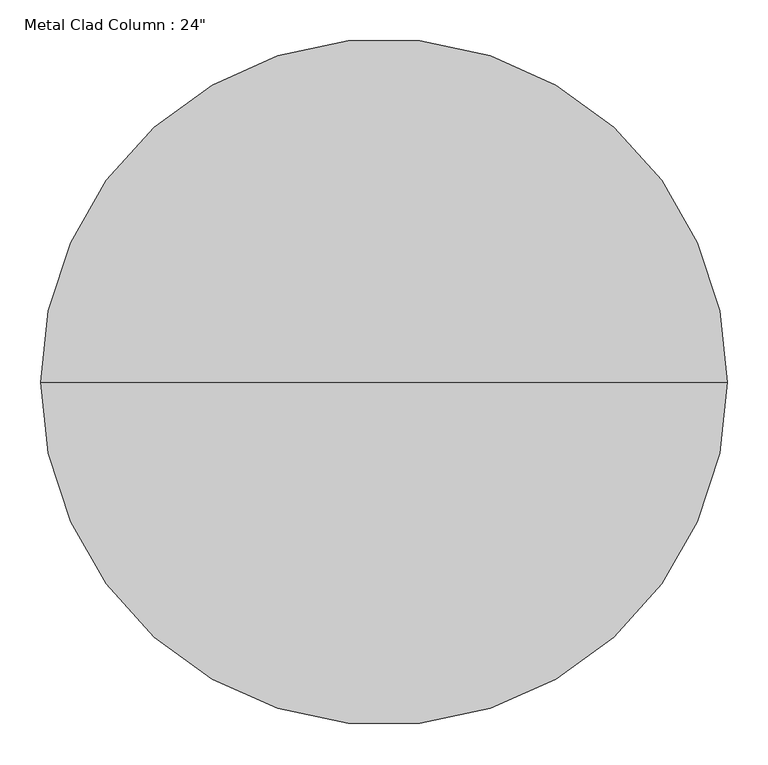
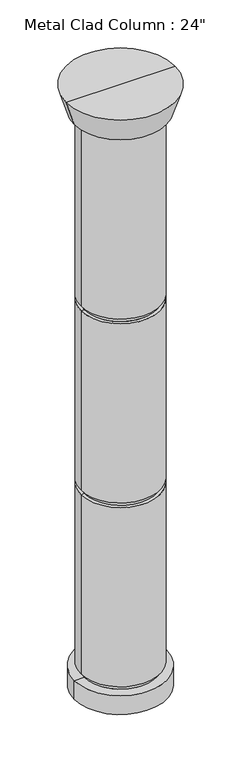
"""IFC4 building model written with IfcOpenShell, lengths in millimetres: column geometry."""

import ifcopenshell
import ifcopenshell.guid

model = None  # the IFC model being written
_history = None  # IfcOwnerHistory: only IFC2X3 demands one
_inside = {}  # id of a spatial element -> (the spatial element, [elements in it])
_under = {}  # id of a project, library or spatial element -> (it, [spatial elements below it])
_declared = {}  # id of a project -> (the project, [libraries it declares])
_typed = {}  # id of a type object -> (the type object, [elements of that type])
_made_of = {}  # id of a material, layer set ... -> (it, [elements and type objects made of it])


def new_model(schema):
    """Start an empty IFC model of exactly this schema.

    Asked for "IFC4X3", IfcOpenShell would pick the latest addendum, in which some entities
    have other attributes; the version numbers below select the first issue.
    IFC2X3 requires an IfcOwnerHistory on every rooted entity: one is made here for all.
    """
    global model, _history
    if schema == "IFC4X3":
        model = ifcopenshell.file(schema_version=(4, 3, 0, 0))
    else:
        model = ifcopenshell.file(schema=schema)
    _inside.clear()
    _under.clear()
    _declared.clear()
    _typed.clear()
    _made_of.clear()
    _history = None
    if model.schema == "IFC2X3":
        org = make("IfcOrganization", Name="unknown")
        user = make(
            "IfcPersonAndOrganization",
            ThePerson=make("IfcPerson", FamilyName="unknown"),
            TheOrganization=org,
        )
        app = make(
            "IfcApplication",
            ApplicationDeveloper=org,
            Version="unknown",
            ApplicationFullName="unknown",
            ApplicationIdentifier="unknown",
        )
        _history = make(
            "IfcOwnerHistory",
            OwningUser=user,
            OwningApplication=app,
            ChangeAction="ADDED",
            CreationDate=0,
        )
    return model


def make(cls, **values):
    """One entity of the class cls with the attributes given. An attribute that is None is left unset."""
    return model.create_entity(
        cls, **{name: value for name, value in values.items() if value is not None}
    )


def rooted(cls, **values):
    """An entity with a GlobalId (a new one), such as an element, a storey or a relation."""
    return make(cls, GlobalId=ifcopenshell.guid.new(), OwnerHistory=_history, **values)


def si_unit(unit_type, name, prefix=None):
    """IfcSIUnit, for example si_unit("LENGTHUNIT", "METRE", prefix="MILLI")."""
    return make("IfcSIUnit", UnitType=unit_type, Prefix=prefix, Name=name)


def assignment(units):
    """IfcUnitAssignment: the units of a project."""
    return None if units is None else make("IfcUnitAssignment", Units=units)


def point(xyz):
    """IfcCartesianPoint."""
    return None if xyz is None else make("IfcCartesianPoint", Coordinates=xyz)


def direction(xyz):
    """IfcDirection."""
    return None if xyz is None else make("IfcDirection", DirectionRatios=xyz)


def frame(location, z_axis=None, x_axis=None):
    """IfcAxis2Placement3D, a coordinate frame: its origin and axes. An axis left out is left unset."""
    return make(
        "IfcAxis2Placement3D",
        Location=point(location),
        Axis=direction(z_axis),
        RefDirection=direction(x_axis),
    )


def origin():
    """The frame at (0, 0, 0) with its axes left unset."""
    return frame((0.0, 0.0, 0.0))


def place(relative_to, where):
    """IfcLocalPlacement: puts the frame where relative to a parent placement (None: the world)."""
    return make(
        "IfcLocalPlacement", PlacementRelTo=relative_to, RelativePlacement=where
    )


def context(
    kind, dimensions, precision=None, world=None, true_north=None, identifier=None
):
    """IfcGeometricRepresentationContext, for example the 3D "Model" context."""
    return make(
        "IfcGeometricRepresentationContext",
        ContextIdentifier=identifier,
        ContextType=kind,
        CoordinateSpaceDimension=dimensions,
        Precision=precision,
        WorldCoordinateSystem=world,
        TrueNorth=true_north,
    )


def project(units=None, contexts=None):
    """IfcProject with its units and contexts."""
    return rooted(
        "IfcProject",
        Name="project",
        RepresentationContexts=contexts,
        UnitsInContext=assignment(units),
    )


def spatial(cls, under=None, at=None, **own):
    """A site, building, storey or space (cls), placed at a placement, below another one or the project."""
    s = rooted(cls, ObjectPlacement=at, **own)
    if under is not None:
        _under.setdefault(under.id(), (under, []))[1].append(s)
    return s


def polyline(points):
    """IfcPolyline through the points."""
    return make("IfcPolyline", Points=[point(p) for p in points])


def circle_curve(where, radius):
    """IfcCircle in the frame where."""
    return make("IfcCircle", Position=where, Radius=radius)


def shape(context_of_items, identifier, shape_type, items):
    """IfcShapeRepresentation: the items that make up one representation, for example the "Body"."""
    return make(
        "IfcShapeRepresentation",
        ContextOfItems=context_of_items,
        RepresentationIdentifier=identifier,
        RepresentationType=shape_type,
        Items=items,
    )


def source(mapping_origin, context_of_items, identifier, shape_type, items):
    """IfcRepresentationMap: a shape defined once, which mapped items show again and again."""
    return make(
        "IfcRepresentationMap",
        MappingOrigin=mapping_origin,
        MappedRepresentation=shape(context_of_items, identifier, shape_type, items),
    )


def transform(
    local_origin,
    x_axis=None,
    y_axis=None,
    z_axis=None,
    scale=None,
    scale2=None,
    scale3=None,
    uniform=True,
):
    """IfcCartesianTransformationOperator3D, or its non-uniform kind. x_axis, y_axis, z_axis: its Axis1, 2, 3."""
    if uniform:
        return make(
            "IfcCartesianTransformationOperator3D",
            Axis1=direction(x_axis),
            Axis2=direction(y_axis),
            LocalOrigin=point(local_origin),
            Scale=scale,
            Axis3=direction(z_axis),
        )
    return make(
        "IfcCartesianTransformationOperator3DnonUniform",
        Axis1=direction(x_axis),
        Axis2=direction(y_axis),
        LocalOrigin=point(local_origin),
        Scale=scale,
        Axis3=direction(z_axis),
        Scale2=scale2,
        Scale3=scale3,
    )


def mapped(mapping_source, mapping_target):
    """IfcMappedItem: shows the shape of a source again, moved by a transform."""
    return make(
        "IfcMappedItem", MappingSource=mapping_source, MappingTarget=mapping_target
    )


def made_of(thing, what):
    """Note that an element or type object is made of a material, layer set ...; save() writes the relation."""
    if what is not None:
        _made_of.setdefault(what.id(), (what, []))[1].append(thing)
    return thing


def element(
    cls,
    number,
    at=None,
    inside=None,
    cuts=None,
    type_object=None,
    material=None,
    context=None,
    identifier="Body",
    shape_type=None,
    held_by="IfcProductDefinitionShape",
    body=None,
    shapes=None,
    **own,
):
    """One element of the class cls, such as IfcWall. Its Tag is "e" and its number.

    at: its placement. inside: the storey or other place that contains it. cuts: it is an
    opening in that element (IfcRelVoidsElement). A single representation is given by context,
    identifier, shape_type and body (its items); several are given by shapes. held_by: the class
    of the entity that holds the representations. save() writes the other relations.
    """
    e = rooted(cls, Tag="e%d" % number, ObjectPlacement=at, **own)
    if body is not None:
        shapes = [shape(context, identifier, shape_type, body)]
    if shapes is not None:
        e.Representation = make(held_by, Representations=shapes)
    if inside is not None:
        _inside.setdefault(inside.id(), (inside, []))[1].append(e)
    if cuts is not None:
        rooted(
            "IfcRelVoidsElement", RelatingBuildingElement=cuts, RelatedOpeningElement=e
        )
    if type_object is not None:
        _typed.setdefault(type_object.id(), (type_object, []))[1].append(e)
    return made_of(e, material)


def aggregate(whole, parts):
    """IfcRelAggregates: a whole, such as a stair, and the parts it consists of."""
    return rooted("IfcRelAggregates", RelatingObject=whole, RelatedObjects=parts)


def save(model, path):
    """Write the relations noted so far, then the file.

    IfcRelAggregates (storeys below a building ...), IfcRelContainedInSpatialStructure (elements
    in a storey), IfcRelDefinesByType, IfcRelAssociatesMaterial and IfcRelDeclares: one each for
    every whole, place, type object, material and project.
    """
    for whole, parts in _under.values():
        aggregate(whole, parts)
    for where, things in _inside.values():
        rooted(
            "IfcRelContainedInSpatialStructure",
            RelatedElements=things,
            RelatingStructure=where,
        )
    for kind, things in _typed.values():
        rooted("IfcRelDefinesByType", RelatedObjects=things, RelatingType=kind)
    for what, things in _made_of.values():
        rooted("IfcRelAssociatesMaterial", RelatedObjects=things, RelatingMaterial=what)
    for by, libraries in _declared.values():
        rooted("IfcRelDeclares", RelatingContext=by, RelatedDefinitions=libraries)
    model.write(path)


def plane_surface(at):
    """IfcPlane: the flat surface through the origin of the frame at, square to its z axis."""
    return make("IfcPlane", Position=at)


def cylinder_surface(at, radius):
    """IfcCylindricalSurface: all points at the distance radius from the z axis of the frame at."""
    return make("IfcCylindricalSurface", Position=at, Radius=radius)


def revolved_surface(curve, axis_point, axis_direction):
    """IfcSurfaceOfRevolution: the curve turned about the line through axis_point along axis_direction."""
    return make(
        "IfcSurfaceOfRevolution",
        SweptCurve=make("IfcArbitraryOpenProfileDef", ProfileType="CURVE", Curve=curve),
        AxisPosition=make("IfcAxis1Placement", Location=point(axis_point), Axis=direction(axis_direction)),
    )


def advanced_brep(points, edges, surfaces, faces):
    """IfcAdvancedBrep: a solid bounded by faces that lie on surfaces and meet in shared edges.

    An edge is (start, end): straight between two places in points (the first is 0);
    or (start, end, curve); or (start, end, curve, False) where it runs against its curve.
    A face is (place in surfaces, loops), or (place, loops, False) where it looks against
    its surface's normal. A loop lists edges by number (the first is 1), with a minus sign
    where the edge is run from its end to its start. The first loop is the outer one.
    """
    corners = [point(p) for p in points]
    vertices = [make("IfcVertexPoint", VertexGeometry=c) for c in corners]
    made = []
    for start, end, *more in edges:
        made.append(
            make(
                "IfcEdgeCurve",
                EdgeStart=vertices[start],
                EdgeEnd=vertices[end],
                EdgeGeometry=more[0] if more else make("IfcPolyline", Points=[corners[start], corners[end]]),
                SameSense=more[1] if len(more) > 1 else True,
            )
        )
    hull = []
    for where, loops, *sense in faces:
        bounds = []
        for j, loop in enumerate(loops):
            ring = [make("IfcOrientedEdge", EdgeElement=made[abs(k) - 1], Orientation=k > 0) for k in loop]
            bounds.append(
                make(
                    "IfcFaceOuterBound" if j == 0 else "IfcFaceBound",
                    Bound=make("IfcEdgeLoop", EdgeList=ring),
                    Orientation=True,
                )
            )
        hull.append(make("IfcAdvancedFace", Bounds=bounds, FaceSurface=surfaces[where], SameSense=sense[0] if sense else True))
    return make("IfcAdvancedBrep", Outer=make("IfcClosedShell", CfsFaces=hull))


def column_9238a582(model_context):
    return source(origin(), model_context, "Body", "AdvancedBrep", [
        advanced_brep(
        [(0.0, 0.0, 0.0), (-355.6, 0.0, 0.0), (355.6, 0.0, 0.0), (-355.6, 0.0, 152.4), (355.6, 0.0, 152.4), (279.4, 0.0, 1684.8666667), (-279.4, 0.0, 1684.8666667), (-304.8, 0.0, 1684.8666667), (304.8, 0.0, 1684.8666667), (-304.8, 0.0, 3141.1333333), (304.8, 0.0, 3141.1333333), (279.4, 0.0, 1646.7666667), (-279.4, 0.0, 1646.7666667), (304.8, 0.0, 1646.7666667), (-304.8, 0.0, 1646.7666667), (304.8, 0.0, 190.5), (-304.8, 0.0, 190.5), (279.4, 0.0, 190.5), (-279.4, 0.0, 190.5), (279.4, 0.0, 152.4), (-279.4, 0.0, 152.4), (355.6, 0.0, 4673.6), (-355.6, 0.0, 4673.6), (-419.1, 0.0, 4876.8), (419.1, 0.0, 4876.8), (0.0, 0.0, 4876.8), (279.4, 0.0, 4673.6), (-279.4, 0.0, 4673.6), (279.4, 0.0, 4635.5), (-279.4, 0.0, 4635.5), (304.8, 0.0, 4635.5), (-304.8, 0.0, 4635.5), (304.8, 0.0, 3179.2333333), (-304.8, 0.0, 3179.2333333), (279.4, 0.0, 3179.2333333), (-279.4, 0.0, 3179.2333333), (279.4, 0.0, 3141.1333333), (-279.4, 0.0, 3141.1333333)],
        [
            (0, 1),
            (1, 2, circle_curve(frame((0.0, 0.0, 0.0), z_axis=(0.0, 0.0, -1.0), x_axis=(-1.0, 0.0, 0.0)), 355.6)),
            (2, 0),
            (2, 1, circle_curve(frame((0.0, 0.0, 0.0), z_axis=(0.0, 0.0, -1.0), x_axis=(-1.0, 0.0, 0.0)), 355.6)),
            (1, 3),
            (3, 4, circle_curve(frame((0.0, 0.0, 152.4), z_axis=(0.0, 0.0, -1.0), x_axis=(-1.0, 0.0, 0.0)), 355.6)),
            (4, 2),
            (4, 3, circle_curve(frame((0.0, 0.0, 152.4), z_axis=(0.0, 0.0, -1.0), x_axis=(-1.0, 0.0, 0.0)), 355.6)),
            (5, 6, circle_curve(frame((0.0, 0.0, 1684.8666667), z_axis=(0.0, 0.0, 1.0), x_axis=(-1.0, 0.0, 0.0)), 279.4)),
            (6, 7),
            (7, 8, circle_curve(frame((0.0, 0.0, 1684.8666667), z_axis=(0.0, 0.0, -1.0), x_axis=(-1.0, 0.0, 0.0)), 304.8)),
            (8, 5),
            (7, 9),
            (9, 10, circle_curve(frame((0.0, 0.0, 3141.1333333), z_axis=(0.0, 0.0, -1.0), x_axis=(-1.0, 0.0, 0.0)), 304.8)),
            (10, 8),
            (7, 8, circle_curve(frame((0.0, 0.0, 1684.8666667), z_axis=(0.0, 0.0, 1.0), x_axis=(-1.0, 0.0, 0.0)), 304.8)),
            (10, 9, circle_curve(frame((0.0, 0.0, 3141.1333333), z_axis=(0.0, 0.0, -1.0), x_axis=(-1.0, 0.0, 0.0)), 304.8)),
            (6, 5, circle_curve(frame((0.0, 0.0, 1684.8666667), z_axis=(0.0, 0.0, 1.0), x_axis=(-1.0, 0.0, 0.0)), 279.4)),
            (11, 12, circle_curve(frame((0.0, 0.0, 1646.7666667), z_axis=(0.0, 0.0, 1.0), x_axis=(-1.0, 0.0, 0.0)), 279.4)),
            (12, 6),
            (5, 11),
            (12, 11, circle_curve(frame((0.0, 0.0, 1646.7666667), z_axis=(0.0, 0.0, 1.0), x_axis=(-1.0, 0.0, 0.0)), 279.4)),
            (13, 14, circle_curve(frame((0.0, 0.0, 1646.7666667), z_axis=(0.0, 0.0, 1.0), x_axis=(-1.0, 0.0, 0.0)), 304.8)),
            (14, 12),
            (11, 13),
            (14, 13, circle_curve(frame((0.0, 0.0, 1646.7666667), z_axis=(0.0, 0.0, 1.0), x_axis=(-1.0, 0.0, 0.0)), 304.8)),
            (15, 16, circle_curve(frame((0.0, 0.0, 190.5), z_axis=(0.0, 0.0, 1.0), x_axis=(-1.0, 0.0, 0.0)), 304.8)),
            (16, 14),
            (13, 15),
            (16, 15, circle_curve(frame((0.0, 0.0, 190.5), z_axis=(0.0, 0.0, 1.0), x_axis=(-1.0, 0.0, 0.0)), 304.8)),
            (17, 18, circle_curve(frame((0.0, 0.0, 190.5), z_axis=(0.0, 0.0, 1.0), x_axis=(-1.0, 0.0, 0.0)), 279.4)),
            (18, 16),
            (15, 17),
            (18, 17, circle_curve(frame((0.0, 0.0, 190.5), z_axis=(0.0, 0.0, 1.0), x_axis=(-1.0, 0.0, 0.0)), 279.4)),
            (19, 20, circle_curve(frame((0.0, 0.0, 152.4), z_axis=(0.0, 0.0, 1.0), x_axis=(-1.0, 0.0, 0.0)), 279.4)),
            (20, 18),
            (17, 19),
            (20, 19, circle_curve(frame((0.0, 0.0, 152.4), z_axis=(0.0, 0.0, 1.0), x_axis=(-1.0, 0.0, 0.0)), 279.4)),
            (3, 20),
            (19, 4),
            (21, 22, circle_curve(frame((0.0, 0.0, 4673.6), z_axis=(0.0, 0.0, 1.0), x_axis=(-1.0, 0.0, 0.0)), 355.6)),
            (22, 23),
            (23, 24, circle_curve(frame((0.0, 0.0, 4876.8), z_axis=(0.0, 0.0, -1.0), x_axis=(-1.0, 0.0, 0.0)), 419.1)),
            (24, 21),
            (23, 25),
            (25, 24),
            (23, 24, circle_curve(frame((0.0, 0.0, 4876.8), z_axis=(0.0, 0.0, 1.0), x_axis=(-1.0, 0.0, 0.0)), 419.1)),
            (22, 21, circle_curve(frame((0.0, 0.0, 4673.6), z_axis=(0.0, 0.0, 1.0), x_axis=(-1.0, 0.0, 0.0)), 355.6)),
            (26, 27, circle_curve(frame((0.0, 0.0, 4673.6), z_axis=(0.0, 0.0, 1.0), x_axis=(-1.0, 0.0, 0.0)), 279.4)),
            (27, 22),
            (21, 26),
            (27, 26, circle_curve(frame((0.0, 0.0, 4673.6), z_axis=(0.0, 0.0, 1.0), x_axis=(-1.0, 0.0, 0.0)), 279.4)),
            (28, 29, circle_curve(frame((0.0, 0.0, 4635.5), z_axis=(0.0, 0.0, 1.0), x_axis=(-1.0, 0.0, 0.0)), 279.4)),
            (29, 27),
            (26, 28),
            (29, 28, circle_curve(frame((0.0, 0.0, 4635.5), z_axis=(0.0, 0.0, 1.0), x_axis=(-1.0, 0.0, 0.0)), 279.4)),
            (30, 31, circle_curve(frame((0.0, 0.0, 4635.5), z_axis=(0.0, 0.0, 1.0), x_axis=(-1.0, 0.0, 0.0)), 304.8)),
            (31, 29),
            (28, 30),
            (31, 30, circle_curve(frame((0.0, 0.0, 4635.5), z_axis=(0.0, 0.0, 1.0), x_axis=(-1.0, 0.0, 0.0)), 304.8)),
            (32, 33, circle_curve(frame((0.0, 0.0, 3179.2333333), z_axis=(0.0, 0.0, 1.0), x_axis=(-1.0, 0.0, 0.0)), 304.8)),
            (33, 31),
            (30, 32),
            (33, 32, circle_curve(frame((0.0, 0.0, 3179.2333333), z_axis=(0.0, 0.0, 1.0), x_axis=(-1.0, 0.0, 0.0)), 304.8)),
            (34, 35, circle_curve(frame((0.0, 0.0, 3179.2333333), z_axis=(0.0, 0.0, 1.0), x_axis=(-1.0, 0.0, 0.0)), 279.4)),
            (35, 33),
            (32, 34),
            (35, 34, circle_curve(frame((0.0, 0.0, 3179.2333333), z_axis=(0.0, 0.0, 1.0), x_axis=(-1.0, 0.0, 0.0)), 279.4)),
            (36, 37, circle_curve(frame((0.0, 0.0, 3141.1333333), z_axis=(0.0, 0.0, 1.0), x_axis=(-1.0, 0.0, 0.0)), 279.4)),
            (37, 35),
            (34, 36),
            (37, 36, circle_curve(frame((0.0, 0.0, 3141.1333333), z_axis=(0.0, 0.0, 1.0), x_axis=(-1.0, 0.0, 0.0)), 279.4)),
            (9, 37),
            (36, 10),
        ],
        [
            plane_surface(frame((0.0, 0.0, 0.0), z_axis=(0.0, 0.0, -1.0), x_axis=(-1.0, 0.0, 0.0))),
            cylinder_surface(frame((0.0, 0.0, 4876.8), z_axis=(0.0, 0.0, -1.0), x_axis=(-1.0, 0.0, 0.0)), 355.6),
            plane_surface(frame((0.0, 0.0, 1684.8666667), z_axis=(0.0, 0.0, -1.0), x_axis=(-1.0, 0.0, 0.0))),
            cylinder_surface(frame((0.0, 0.0, 4876.8), z_axis=(0.0, 0.0, -1.0), x_axis=(-1.0, 0.0, 0.0)), 304.8),
            cylinder_surface(frame((0.0, 0.0, 4876.8), z_axis=(0.0, 0.0, -1.0), x_axis=(-1.0, 0.0, 0.0)), 279.4),
            plane_surface(frame((0.0, 0.0, 1646.7666667), z_axis=(0.0, 0.0, 1.0), x_axis=(-1.0, 0.0, 0.0))),
            plane_surface(frame((0.0, 0.0, 190.5), z_axis=(0.0, 0.0, -1.0), x_axis=(-1.0, 0.0, 0.0))),
            plane_surface(frame((0.0, 0.0, 152.4), z_axis=(0.0, 0.0, 1.0), x_axis=(-1.0, 0.0, 0.0))),
            revolved_surface(polyline([(-419.1, 0.0, 4876.8), (-355.6, 0.0, 4673.6)]), (0.0, 0.0, 4876.8), (0.0, 0.0, -1.0)),
            plane_surface(frame((0.0, 0.0, 4876.8), z_axis=(0.0, 0.0, 1.0), x_axis=(-1.0, 0.0, 0.0))),
            plane_surface(frame((0.0, 0.0, 4673.6), z_axis=(0.0, 0.0, -1.0), x_axis=(-1.0, 0.0, 0.0))),
            plane_surface(frame((0.0, 0.0, 4635.5), z_axis=(0.0, 0.0, 1.0), x_axis=(-1.0, 0.0, 0.0))),
            plane_surface(frame((0.0, 0.0, 3179.2333333), z_axis=(0.0, 0.0, -1.0), x_axis=(-1.0, 0.0, 0.0))),
            plane_surface(frame((0.0, 0.0, 3141.1333333), z_axis=(0.0, 0.0, 1.0), x_axis=(-1.0, 0.0, 0.0))),
        ],
        [
            (0, [[1, 2, 3]]),
            (0, [[-3, 4, -1]]),
            (1, [[-2, 5, 6, 7]]),
            (1, [[-4, -7, 8, -5]]),
            (2, [[9, 10, 11, 12]]),
            (3, [[-11, 13, 14, 15]]),
            (3, [[16, -15, 17, -13]]),
            (2, [[18, -12, -16, -10]]),
            (4, [[19, 20, -9, 21]]),
            (4, [[22, -21, -18, -20]]),
            (5, [[23, 24, -19, 25]]),
            (5, [[26, -25, -22, -24]]),
            (3, [[27, 28, -23, 29]]),
            (3, [[30, -29, -26, -28]]),
            (6, [[31, 32, -27, 33]]),
            (6, [[34, -33, -30, -32]]),
            (4, [[35, 36, -31, 37]]),
            (4, [[38, -37, -34, -36]]),
            (7, [[-6, 39, -35, 40]]),
            (7, [[-8, -40, -38, -39]]),
            (8, [[41, 42, 43, 44]]),
            (9, [[-43, 45, 46]]),
            (9, [[47, -46, -45]]),
            (8, [[48, -44, -47, -42]]),
            (10, [[49, 50, -41, 51]]),
            (10, [[52, -51, -48, -50]]),
            (4, [[53, 54, -49, 55]]),
            (4, [[56, -55, -52, -54]]),
            (11, [[57, 58, -53, 59]]),
            (11, [[60, -59, -56, -58]]),
            (3, [[61, 62, -57, 63]]),
            (3, [[64, -63, -60, -62]]),
            (12, [[65, 66, -61, 67]]),
            (12, [[68, -67, -64, -66]]),
            (4, [[69, 70, -65, 71]]),
            (4, [[72, -71, -68, -70]]),
            (13, [[-14, 73, -69, 74]]),
            (13, [[-17, -74, -72, -73]]),
        ],
    ),
    ])


if __name__ == "__main__":
    model = new_model("IFC4")
    model_context = context("Model", 3, world=origin())
    ifc_project = project(units=[si_unit("LENGTHUNIT", "METRE", prefix="MILLI")], contexts=[model_context])
    site = spatial("IfcSite", under=ifc_project)
    building = spatial("IfcBuilding", under=site)
    placement = place(None, origin())
    column_shape = column_9238a582(model_context)
    element("IfcColumn", 1, ObjectType="Metal Clad Column : 24\"", at=placement, inside=building, context=model_context, shape_type="MappedRepresentation", body=[
        mapped(column_shape, transform((0.0, 0.0, 0.0), x_axis=(1.0, 0.0, 0.0), y_axis=(0.0, 1.0, 0.0), z_axis=(0.0, 0.0, 1.0))),
    ])
    save(model, "model.ifc")

# Revit data of these elements
# Type "Metal Clad Column : 24\""
#   Assembly Code = "B1010200"
#   Base = 0' - 6"
#   Capital = 0' - 8"
#   Diameter = 2' - 0"
#   Joint Depth = 0' - 1"
#   Joint Width = 0' - 1 1/2"
#   Offset base level = 0' - 0"
#   Offset top level = 0' - 0"
#   Material = Aluminum
# Element 1 (IfcColumn, "Metal Clad Column : 24\"")
#   Materials on its faces: "Aluminum"
# Materials
#   "Aluminum": class "Metal", colour RGB 247 247 247, transparency 0, Description = "Aluminum 6061", Cost = 0
